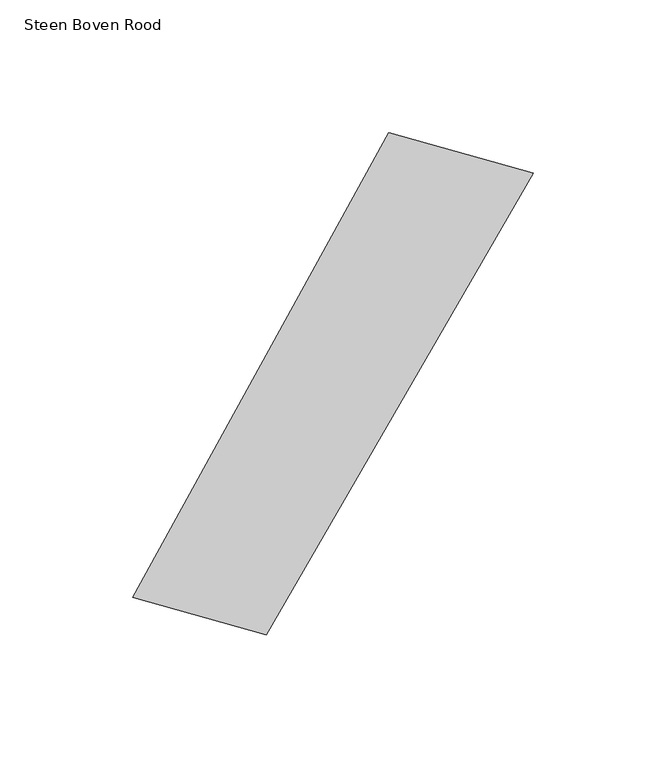
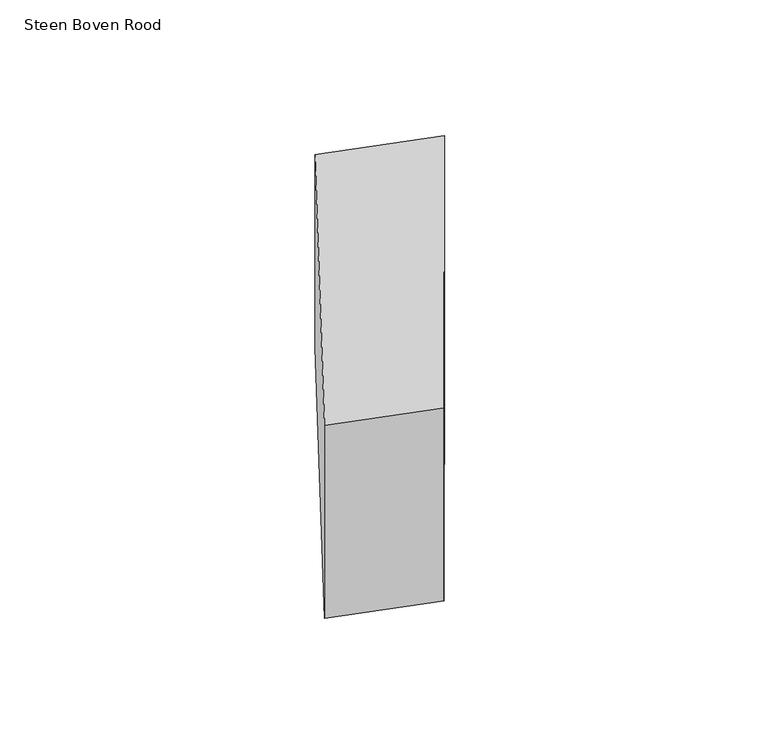
"""IFC4 building model written with IfcOpenShell, lengths in millimetres: proxy geometry, 00_GMA_steen_versie_4 : Steen Boven Rood."""

from ifc_helpers import new_model, si_unit, origin, origin_with_axes, place, context, project, spatial, polyline, outline, extrude, source, transform, mapped, element, save


def steen_boven_rood_b5eb2da5(model_context):
    return source(origin(), model_context, "Body", "SweptSolid", [
        extrude(outline(polyline([(152.4101366, 159.2988443), (51.5730688, -15.069089), (1.2080744, -0.8854472), (97.8590073, 174.6378601), (152.4101366, 159.2988443)])), origin_with_axes(), (0.0, 0.0, 1.0), 100.0),
    ])


if __name__ == "__main__":
    model = new_model("IFC4")
    model_context = context("Model", 3, world=origin())
    ifc_project = project(units=[si_unit("LENGTHUNIT", "METRE", prefix="MILLI")], contexts=[model_context])
    site = spatial("IfcSite", under=ifc_project)
    building = spatial("IfcBuilding", under=site)
    placement = place(None, origin())
    steen_boven_rood_shape = steen_boven_rood_b5eb2da5(model_context)
    element("IfcBuildingElementProxy", 1, Name="00_GMA_steen_versie_4 : Steen Boven Rood", ObjectType="00_GMA_steen_versie_4 : Steen Boven Rood", at=placement, inside=building, context=model_context, shape_type="MappedRepresentation", body=[
        mapped(steen_boven_rood_shape, transform((0.0, 0.0, 0.0), x_axis=(1.0, 0.0, 0.0), y_axis=(0.0, 1.0, 0.0), z_axis=(0.0, 0.0, 1.0))),
    ])
    save(model, "model.ifc")

# Revit data of these elements
# Type "00_GMA_steen_versie_4 : Steen Boven Rood"
#   StootVoegHalfBoven [instance default] = 5 mm
#   StootVoegHalf [instance default] = 5 mm
#   StootVoegBreedteOnder = 10 mm
#   StootVoegBreedteBoven = 10 mm
#   Steendikte = 100 mm
#   LintVoegOnderHalf = 5 mm
#   LintVoegOnder = 10 mm
#   LintVoegBovenHalf = 0 mm
#   LintVoegBoven = 0 mm
#   materiaal = 21_steen_rood
#   MateriaalVoeg = none
#   Default Elevation = 0
# Element 1 (IfcBuildingElementProxy, "00_GMA_steen_versie_4 : Steen Boven Rood")
#   Materials on its faces: "21_steen_rood"
# Materials
#   "21_steen_rood": class "Unassigned", colour RGB 213 111 43, transparency 0, Cost = 0
